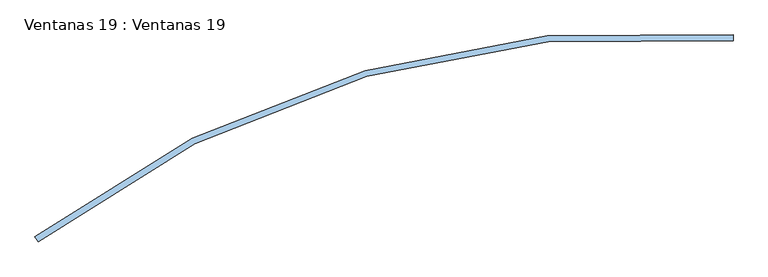
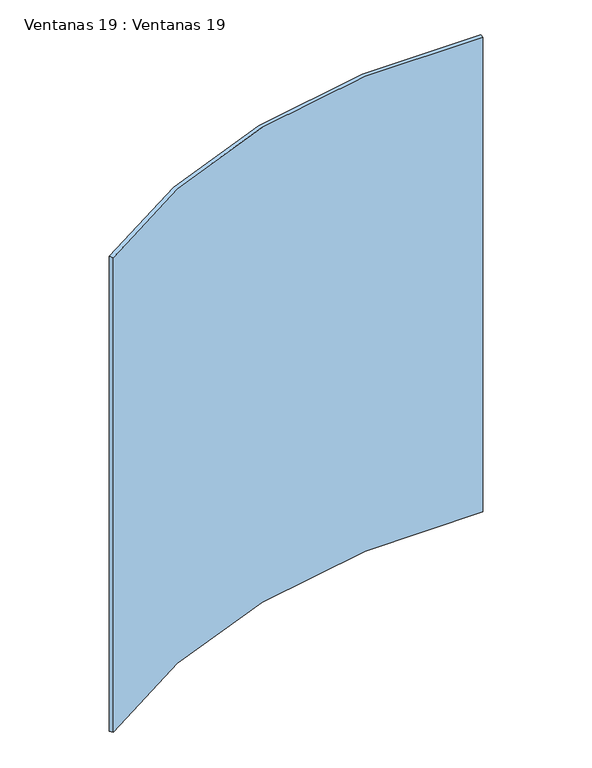
"""IFC4 building model written with IfcOpenShell, lengths in millimetres: window geometry, Ventanas 19 : Ventanas 19."""

from ifc_helpers import new_model, si_unit, point, frame, frame_2d, origin, place, context, project, spatial, polyline, circle_curve, trimmed, segment, composite_curve, outline, extrude, source, transform, mapped, element, save


def ventanas_19_ventanas_19_27d367e9(model_context):
    return source(origin(), model_context, "Body", "SweptSolid", [
        extrude(outline(composite_curve([segment(polyline([(-5154.373754, 11159.8353841), (-5154.373754, 11139.8353841)]), True, "CONTINUOUS"), segment(trimmed(circle_curve(frame_2d((-5454.6843622, 7752.5217497)), 3400.5999646), [point((-5154.373754, 11139.8353841))], [point((-7516.6829874, 10456.6374627))], True, "CARTESIAN"), True, "CONTINUOUS"), segment(polyline([(-7516.6829874, 10456.6374627), (-7528.1545162, 10473.0205035)]), True, "CONTINUOUS"), segment(trimmed(circle_curve(frame_2d((-5454.9594533, 7753.1672859)), 3419.9034042), [point((-7528.1545162, 10473.0205035))], [point((-5154.373754, 11159.8353841))], False, "CARTESIAN"), True, "CONTINUOUS")], self_intersect=False)), frame((0.0, 0.0, 5926.25), z_axis=(0.0, 0.0, 1.0), x_axis=(1.0, 0.0, 0.0)), (0.0, 0.0, 1.0), 2673.75),
    ])


if __name__ == "__main__":
    model = new_model("IFC4")
    model_context = context("Model", 3, world=origin())
    ifc_project = project(units=[si_unit("LENGTHUNIT", "METRE", prefix="MILLI")], contexts=[model_context])
    site = spatial("IfcSite", under=ifc_project)
    building = spatial("IfcBuilding", under=site)
    placement = place(None, origin())
    ventanas_19_ventanas_19_shape = ventanas_19_ventanas_19_27d367e9(model_context)
    element("IfcWindow", 1, ObjectType="Ventanas 19 : Ventanas 19", at=placement, inside=building, context=model_context, shape_type="MappedRepresentation", body=[
        mapped(ventanas_19_ventanas_19_shape, transform((0.0, 0.0, 0.0), x_axis=(1.0, 0.0, 0.0), y_axis=(0.0, 1.0, 0.0), z_axis=(0.0, 0.0, 1.0))),
    ])
    save(model, "model.ifc")

# Revit data of these elements
# Type "Ventanas 19 : Ventanas 19"
#   Type Mark = "45"
# Element 1 (IfcWindow, "Ventanas 19 : Ventanas 19")
#   Materials on its faces: "VIDRIO"
# Materials
#   "VIDRIO": class "Genérico", colour RGB 120 120 120, transparency 0, Cost = 0
